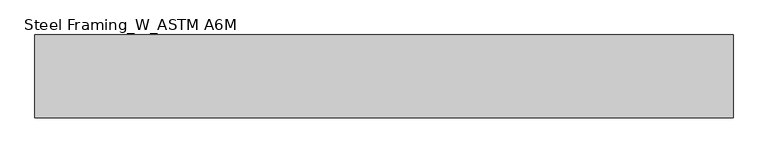
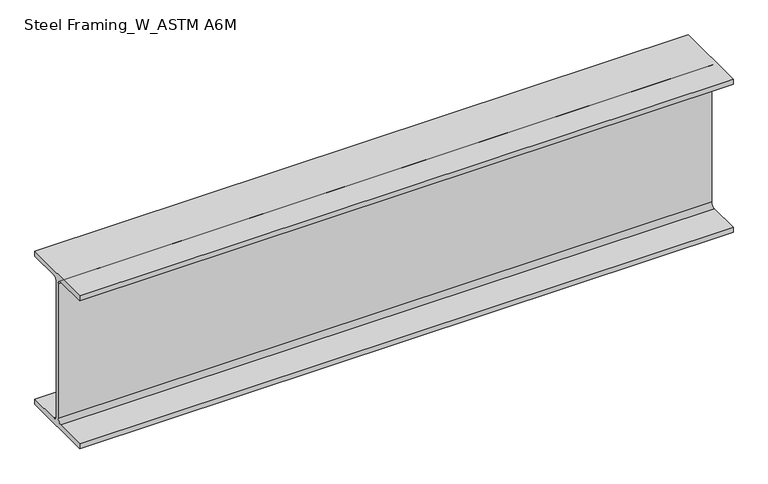
"""IFC4 building model written with IfcOpenShell, lengths in millimetres: beam geometry, Steel Framing_W_ASTM A6M : H_SB_AR_S02_W360x51_G3."""

import ifcopenshell
import ifcopenshell.guid

model = None  # the IFC model being written
_history = None  # IfcOwnerHistory: only IFC2X3 demands one
_inside = {}  # id of a spatial element -> (the spatial element, [elements in it])
_under = {}  # id of a project, library or spatial element -> (it, [spatial elements below it])
_declared = {}  # id of a project -> (the project, [libraries it declares])
_typed = {}  # id of a type object -> (the type object, [elements of that type])
_made_of = {}  # id of a material, layer set ... -> (it, [elements and type objects made of it])


def new_model(schema):
    """Start an empty IFC model of exactly this schema.

    Asked for "IFC4X3", IfcOpenShell would pick the latest addendum, in which some entities
    have other attributes; the version numbers below select the first issue.
    IFC2X3 requires an IfcOwnerHistory on every rooted entity: one is made here for all.
    """
    global model, _history
    if schema == "IFC4X3":
        model = ifcopenshell.file(schema_version=(4, 3, 0, 0))
    else:
        model = ifcopenshell.file(schema=schema)
    _inside.clear()
    _under.clear()
    _declared.clear()
    _typed.clear()
    _made_of.clear()
    _history = None
    if model.schema == "IFC2X3":
        org = make("IfcOrganization", Name="unknown")
        user = make(
            "IfcPersonAndOrganization",
            ThePerson=make("IfcPerson", FamilyName="unknown"),
            TheOrganization=org,
        )
        app = make(
            "IfcApplication",
            ApplicationDeveloper=org,
            Version="unknown",
            ApplicationFullName="unknown",
            ApplicationIdentifier="unknown",
        )
        _history = make(
            "IfcOwnerHistory",
            OwningUser=user,
            OwningApplication=app,
            ChangeAction="ADDED",
            CreationDate=0,
        )
    return model


def make(cls, **values):
    """One entity of the class cls with the attributes given. An attribute that is None is left unset."""
    return model.create_entity(
        cls, **{name: value for name, value in values.items() if value is not None}
    )


def rooted(cls, **values):
    """An entity with a GlobalId (a new one), such as an element, a storey or a relation."""
    return make(cls, GlobalId=ifcopenshell.guid.new(), OwnerHistory=_history, **values)


def si_unit(unit_type, name, prefix=None):
    """IfcSIUnit, for example si_unit("LENGTHUNIT", "METRE", prefix="MILLI")."""
    return make("IfcSIUnit", UnitType=unit_type, Prefix=prefix, Name=name)


def assignment(units):
    """IfcUnitAssignment: the units of a project."""
    return None if units is None else make("IfcUnitAssignment", Units=units)


def point(xyz):
    """IfcCartesianPoint."""
    return None if xyz is None else make("IfcCartesianPoint", Coordinates=xyz)


def direction(xyz):
    """IfcDirection."""
    return None if xyz is None else make("IfcDirection", DirectionRatios=xyz)


def frame(location, z_axis=None, x_axis=None):
    """IfcAxis2Placement3D, a coordinate frame: its origin and axes. An axis left out is left unset."""
    return make(
        "IfcAxis2Placement3D",
        Location=point(location),
        Axis=direction(z_axis),
        RefDirection=direction(x_axis),
    )


def frame_2d(location, x_axis=None):
    """IfcAxis2Placement2D, a coordinate frame in the plane: its origin and x axis."""
    return make(
        "IfcAxis2Placement2D", Location=point(location), RefDirection=direction(x_axis)
    )


def origin():
    """The frame at (0, 0, 0) with its axes left unset."""
    return frame((0.0, 0.0, 0.0))


def place(relative_to, where):
    """IfcLocalPlacement: puts the frame where relative to a parent placement (None: the world)."""
    return make(
        "IfcLocalPlacement", PlacementRelTo=relative_to, RelativePlacement=where
    )


def context(
    kind, dimensions, precision=None, world=None, true_north=None, identifier=None
):
    """IfcGeometricRepresentationContext, for example the 3D "Model" context."""
    return make(
        "IfcGeometricRepresentationContext",
        ContextIdentifier=identifier,
        ContextType=kind,
        CoordinateSpaceDimension=dimensions,
        Precision=precision,
        WorldCoordinateSystem=world,
        TrueNorth=true_north,
    )


def project(units=None, contexts=None):
    """IfcProject with its units and contexts."""
    return rooted(
        "IfcProject",
        Name="project",
        RepresentationContexts=contexts,
        UnitsInContext=assignment(units),
    )


def spatial(cls, under=None, at=None, **own):
    """A site, building, storey or space (cls), placed at a placement, below another one or the project."""
    s = rooted(cls, ObjectPlacement=at, **own)
    if under is not None:
        _under.setdefault(under.id(), (under, []))[1].append(s)
    return s


def polyline(points):
    """IfcPolyline through the points."""
    return make("IfcPolyline", Points=[point(p) for p in points])


def circle_curve(where, radius):
    """IfcCircle in the frame where."""
    return make("IfcCircle", Position=where, Radius=radius)


def trimmed(basis, trim1, trim2, sense, master):
    """IfcTrimmedCurve: the piece of a basis curve between two trims."""
    return make(
        "IfcTrimmedCurve",
        BasisCurve=basis,
        Trim1=trim1,
        Trim2=trim2,
        SenseAgreement=sense,
        MasterRepresentation=master,
    )


def segment(curve, same_sense, transition):
    """IfcCompositeCurveSegment."""
    return make(
        "IfcCompositeCurveSegment",
        Transition=transition,
        SameSense=same_sense,
        ParentCurve=curve,
    )


def composite_curve(segments, self_intersect=None):
    """IfcCompositeCurve: segments joined end to end."""
    return make("IfcCompositeCurve", Segments=segments, SelfIntersect=self_intersect)


def outline(outer, holes=None, kind="AREA"):
    """IfcArbitraryClosedProfileDef: a profile drawn as a closed curve; with holes, ...WithVoids."""
    if holes is None:
        return make("IfcArbitraryClosedProfileDef", ProfileType=kind, OuterCurve=outer)
    return make(
        "IfcArbitraryProfileDefWithVoids",
        ProfileType=kind,
        OuterCurve=outer,
        InnerCurves=holes,
    )


def extrude(swept, where, along, depth):
    """IfcExtrudedAreaSolid: the profile swept, set in the frame where, extruded along a direction by depth."""
    return make(
        "IfcExtrudedAreaSolid",
        SweptArea=swept,
        Position=where,
        ExtrudedDirection=direction(along),
        Depth=depth,
    )


def shape(context_of_items, identifier, shape_type, items):
    """IfcShapeRepresentation: the items that make up one representation, for example the "Body"."""
    return make(
        "IfcShapeRepresentation",
        ContextOfItems=context_of_items,
        RepresentationIdentifier=identifier,
        RepresentationType=shape_type,
        Items=items,
    )


def source(mapping_origin, context_of_items, identifier, shape_type, items):
    """IfcRepresentationMap: a shape defined once, which mapped items show again and again."""
    return make(
        "IfcRepresentationMap",
        MappingOrigin=mapping_origin,
        MappedRepresentation=shape(context_of_items, identifier, shape_type, items),
    )


def transform(
    local_origin,
    x_axis=None,
    y_axis=None,
    z_axis=None,
    scale=None,
    scale2=None,
    scale3=None,
    uniform=True,
):
    """IfcCartesianTransformationOperator3D, or its non-uniform kind. x_axis, y_axis, z_axis: its Axis1, 2, 3."""
    if uniform:
        return make(
            "IfcCartesianTransformationOperator3D",
            Axis1=direction(x_axis),
            Axis2=direction(y_axis),
            LocalOrigin=point(local_origin),
            Scale=scale,
            Axis3=direction(z_axis),
        )
    return make(
        "IfcCartesianTransformationOperator3DnonUniform",
        Axis1=direction(x_axis),
        Axis2=direction(y_axis),
        LocalOrigin=point(local_origin),
        Scale=scale,
        Axis3=direction(z_axis),
        Scale2=scale2,
        Scale3=scale3,
    )


def mapped(mapping_source, mapping_target):
    """IfcMappedItem: shows the shape of a source again, moved by a transform."""
    return make(
        "IfcMappedItem", MappingSource=mapping_source, MappingTarget=mapping_target
    )


def made_of(thing, what):
    """Note that an element or type object is made of a material, layer set ...; save() writes the relation."""
    if what is not None:
        _made_of.setdefault(what.id(), (what, []))[1].append(thing)
    return thing


def element(
    cls,
    number,
    at=None,
    inside=None,
    cuts=None,
    type_object=None,
    material=None,
    context=None,
    identifier="Body",
    shape_type=None,
    held_by="IfcProductDefinitionShape",
    body=None,
    shapes=None,
    **own,
):
    """One element of the class cls, such as IfcWall. Its Tag is "e" and its number.

    at: its placement. inside: the storey or other place that contains it. cuts: it is an
    opening in that element (IfcRelVoidsElement). A single representation is given by context,
    identifier, shape_type and body (its items); several are given by shapes. held_by: the class
    of the entity that holds the representations. save() writes the other relations.
    """
    e = rooted(cls, Tag="e%d" % number, ObjectPlacement=at, **own)
    if body is not None:
        shapes = [shape(context, identifier, shape_type, body)]
    if shapes is not None:
        e.Representation = make(held_by, Representations=shapes)
    if inside is not None:
        _inside.setdefault(inside.id(), (inside, []))[1].append(e)
    if cuts is not None:
        rooted(
            "IfcRelVoidsElement", RelatingBuildingElement=cuts, RelatedOpeningElement=e
        )
    if type_object is not None:
        _typed.setdefault(type_object.id(), (type_object, []))[1].append(e)
    return made_of(e, material)


def aggregate(whole, parts):
    """IfcRelAggregates: a whole, such as a stair, and the parts it consists of."""
    return rooted("IfcRelAggregates", RelatingObject=whole, RelatedObjects=parts)


def save(model, path):
    """Write the relations noted so far, then the file.

    IfcRelAggregates (storeys below a building ...), IfcRelContainedInSpatialStructure (elements
    in a storey), IfcRelDefinesByType, IfcRelAssociatesMaterial and IfcRelDeclares: one each for
    every whole, place, type object, material and project.
    """
    for whole, parts in _under.values():
        aggregate(whole, parts)
    for where, things in _inside.values():
        rooted(
            "IfcRelContainedInSpatialStructure",
            RelatedElements=things,
            RelatingStructure=where,
        )
    for kind, things in _typed.values():
        rooted("IfcRelDefinesByType", RelatedObjects=things, RelatingType=kind)
    for what, things in _made_of.values():
        rooted("IfcRelAssociatesMaterial", RelatedObjects=things, RelatingMaterial=what)
    for by, libraries in _declared.values():
        rooted("IfcRelDeclares", RelatingContext=by, RelatedDefinitions=libraries)
    model.write(path)


def steel_framing_w_astm_a6m_0ec37d14(model_context):
    return source(origin(), model_context, "Body", "SweptSolid", [
        extrude(outline(composite_curve([segment(polyline([(85.5, -166.4), (85.5, -178.0), (-85.5, -178.0), (-85.5, -166.4), (-13.72, -166.4)]), True, "CONTINUOUS"), segment(trimmed(circle_curve(frame_2d((-13.72, -156.3)), 10.1), [point((-13.72, -166.4))], [point((-3.62, -156.3))], True, "CARTESIAN"), True, "CONTINUOUS"), segment(polyline([(-3.62, -156.3), (-3.62, 156.3)]), True, "CONTINUOUS"), segment(trimmed(circle_curve(frame_2d((-13.72, 156.3)), 10.1), [point((-3.62, 156.3))], [point((-13.72, 166.4))], True, "CARTESIAN"), True, "CONTINUOUS"), segment(polyline([(-13.72, 166.4), (-85.5, 166.4), (-85.5, 178.0), (85.5, 178.0), (85.5, 166.4), (13.72, 166.4)]), True, "CONTINUOUS"), segment(trimmed(circle_curve(frame_2d((13.72, 156.3)), 10.1), [point((13.72, 166.4))], [point((3.62, 156.3))], True, "CARTESIAN"), True, "CONTINUOUS"), segment(polyline([(3.62, 156.3), (3.62, -156.3)]), True, "CONTINUOUS"), segment(trimmed(circle_curve(frame_2d((13.72, -156.3)), 10.1), [point((3.62, -156.3))], [point((13.72, -166.4))], True, "CARTESIAN"), True, "CONTINUOUS"), segment(polyline([(13.72, -166.4), (85.5, -166.4)]), True, "CONTINUOUS")], self_intersect=False)), frame((-553.8, 0.0, 0.0), z_axis=(1.0, 0.0, 0.0), x_axis=(0.0, 1.0, 0.0)), (0.0, 0.0, 1.0), 1439.3),
    ])


if __name__ == "__main__":
    model = new_model("IFC4")
    model_context = context("Model", 3, world=origin())
    ifc_project = project(units=[si_unit("LENGTHUNIT", "METRE", prefix="MILLI")], contexts=[model_context])
    site = spatial("IfcSite", under=ifc_project)
    building = spatial("IfcBuilding", under=site)
    placement = place(None, origin())
    steel_framing_w_astm_a6m_shape = steel_framing_w_astm_a6m_0ec37d14(model_context)
    element("IfcBeam", 1, ObjectType="Steel Framing_W_ASTM A6M : H_SB_AR_S02_W360x51_G3", at=placement, inside=building, context=model_context, shape_type="MappedRepresentation", body=[
        mapped(steel_framing_w_astm_a6m_shape, transform((0.0, 0.0, 0.0), x_axis=(1.0, 0.0, 0.0), y_axis=(0.0, 1.0, 0.0), z_axis=(0.0, 0.0, 1.0))),
    ])
    save(model, "model.ifc")

# Revit data of these elements
# Type "Steel Framing_W_ASTM A6M : H_SB_AR_S02_W360x51_G3"
#   Type Mark = "G3"
#   Section Name Key = "W14x34"
#   Width = 17.1 cm
#   Web Thickness = 0.724 cm
#   Web Fillet = 1.01 cm
#   Warping Constant = 287000.0 cm⁶
#   Torsional Moment of Inertia = 23.70 cm⁴
#   Section Area = 64.5 cm²
#   Plastic Modulus weak axis = 174.0 cm³
#   Plastic Modulus strong axis = 895.0 cm³
#   Perimeter = 1.36 m²/m
#   Nominal Weight = 51.00 kgf/m
#   Moment of Inertia weak axis = 970.00 cm⁴
#   Moment of Inertia strong axis = 14200.00 cm⁴
#   Height = 35.6 cm
#   Flange Thickness = 1.16 cm
#   Elastic Modulus weak axis = 113.0 cm³
#   Elastic Modulus strong axis = 796.0 cm³
#   Centroid Vertical = 17.8 cm
#   Centroid Horizontal = 8.55 cm
#   Length [instance default] = 1500 mm
#   Structural Material [instance default] = Steel, 45-345
#   Bolt Spacing = 0
#   Assembly Code = ""
# Element 1 (IfcBeam, "Steel Framing_W_ASTM A6M : H_SB_AR_S02_W360x51_G3")
#   Materials on its faces: "Steel, 45-345"
# Materials
#   "Steel, 45-345": class "Metal", colour RGB 189 187 185, transparency 0, Description = "Steel 345 MPa", Cost = 0
